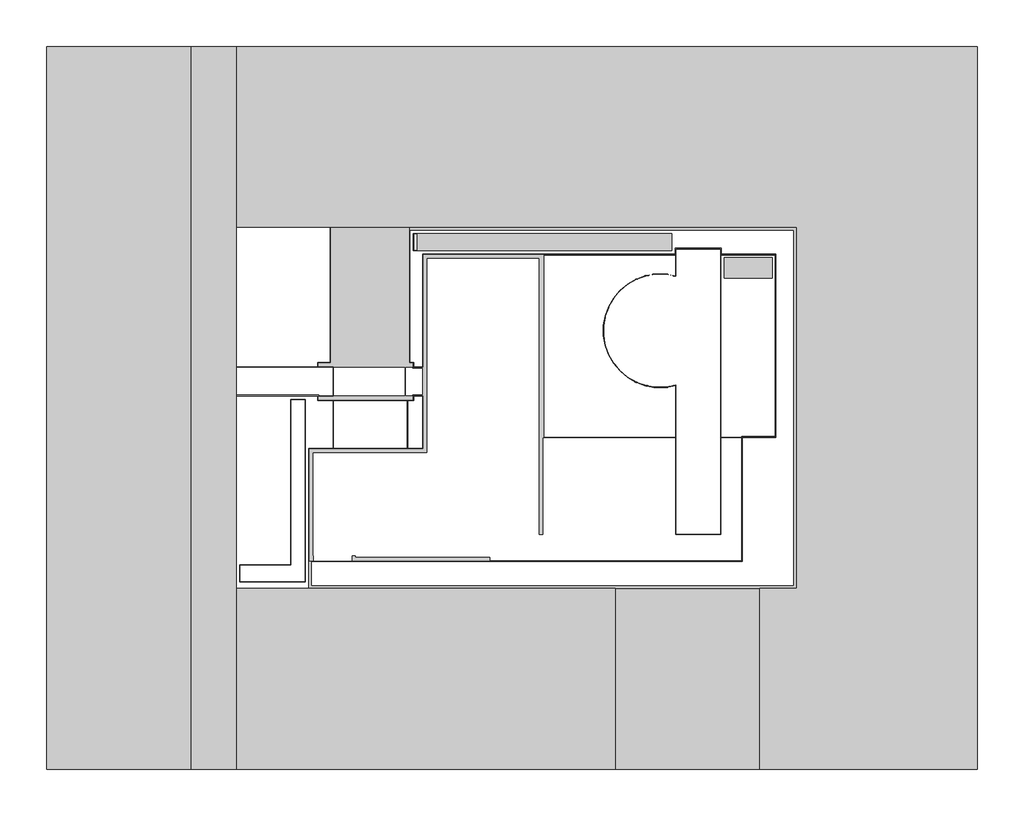
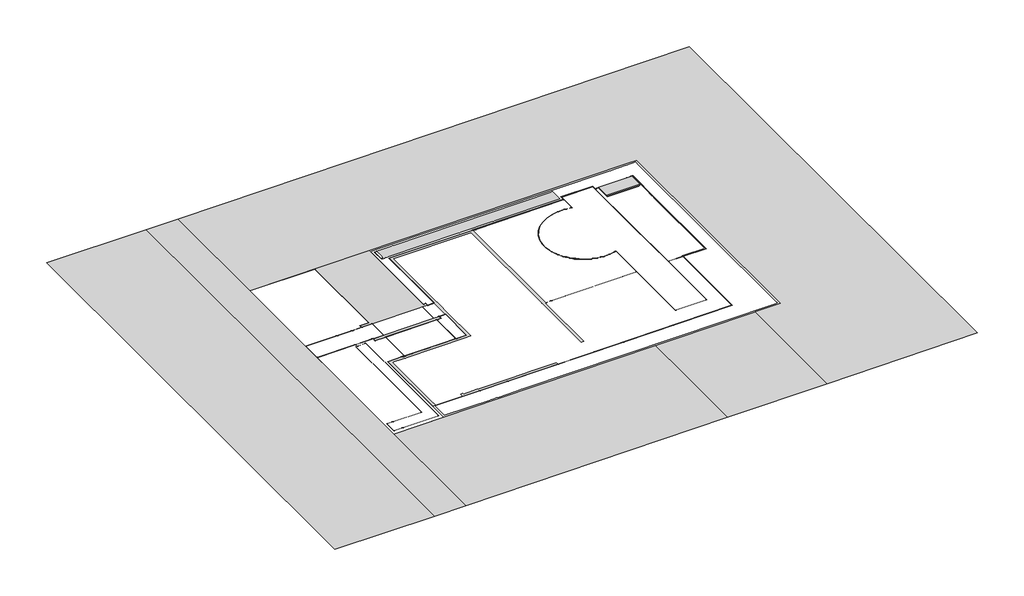
# One storey: 11 proxies.
"""IFC4 building model written with IfcOpenShell, lengths in millimetres."""

import ifcopenshell
import ifcopenshell.guid

model = None  # the IFC model being written
_history = None  # IfcOwnerHistory: only IFC2X3 demands one
_inside = {}  # id of a spatial element -> (the spatial element, [elements in it])
_under = {}  # id of a project, library or spatial element -> (it, [spatial elements below it])
_declared = {}  # id of a project -> (the project, [libraries it declares])
_typed = {}  # id of a type object -> (the type object, [elements of that type])
_made_of = {}  # id of a material, layer set ... -> (it, [elements and type objects made of it])


def new_model(schema):
    """Start an empty IFC model of exactly this schema.

    Asked for "IFC4X3", IfcOpenShell would pick the latest addendum, in which some entities
    have other attributes; the version numbers below select the first issue.
    IFC2X3 requires an IfcOwnerHistory on every rooted entity: one is made here for all.
    """
    global model, _history
    if schema == "IFC4X3":
        model = ifcopenshell.file(schema_version=(4, 3, 0, 0))
    else:
        model = ifcopenshell.file(schema=schema)
    _inside.clear()
    _under.clear()
    _declared.clear()
    _typed.clear()
    _made_of.clear()
    _history = None
    if model.schema == "IFC2X3":
        org = make("IfcOrganization", Name="unknown")
        user = make(
            "IfcPersonAndOrganization",
            ThePerson=make("IfcPerson", FamilyName="unknown"),
            TheOrganization=org,
        )
        app = make(
            "IfcApplication",
            ApplicationDeveloper=org,
            Version="unknown",
            ApplicationFullName="unknown",
            ApplicationIdentifier="unknown",
        )
        _history = make(
            "IfcOwnerHistory",
            OwningUser=user,
            OwningApplication=app,
            ChangeAction="ADDED",
            CreationDate=0,
        )
    return model


def make(cls, **values):
    """One entity of the class cls with the attributes given. An attribute that is None is left unset."""
    return model.create_entity(
        cls, **{name: value for name, value in values.items() if value is not None}
    )


def rooted(cls, **values):
    """An entity with a GlobalId (a new one), such as an element, a storey or a relation."""
    return make(cls, GlobalId=ifcopenshell.guid.new(), OwnerHistory=_history, **values)


def si_unit(unit_type, name, prefix=None):
    """IfcSIUnit, for example si_unit("LENGTHUNIT", "METRE", prefix="MILLI")."""
    return make("IfcSIUnit", UnitType=unit_type, Prefix=prefix, Name=name)


def assignment(units):
    """IfcUnitAssignment: the units of a project."""
    return None if units is None else make("IfcUnitAssignment", Units=units)


def point(xyz):
    """IfcCartesianPoint."""
    return None if xyz is None else make("IfcCartesianPoint", Coordinates=xyz)


def direction(xyz):
    """IfcDirection."""
    return None if xyz is None else make("IfcDirection", DirectionRatios=xyz)


def frame(location, z_axis=None, x_axis=None):
    """IfcAxis2Placement3D, a coordinate frame: its origin and axes. An axis left out is left unset."""
    return make(
        "IfcAxis2Placement3D",
        Location=point(location),
        Axis=direction(z_axis),
        RefDirection=direction(x_axis),
    )


def origin():
    """The frame at (0, 0, 0) with its axes left unset."""
    return frame((0.0, 0.0, 0.0))


def place(relative_to, where):
    """IfcLocalPlacement: puts the frame where relative to a parent placement (None: the world)."""
    return make(
        "IfcLocalPlacement", PlacementRelTo=relative_to, RelativePlacement=where
    )


def context(
    kind, dimensions, precision=None, world=None, true_north=None, identifier=None
):
    """IfcGeometricRepresentationContext, for example the 3D "Model" context."""
    return make(
        "IfcGeometricRepresentationContext",
        ContextIdentifier=identifier,
        ContextType=kind,
        CoordinateSpaceDimension=dimensions,
        Precision=precision,
        WorldCoordinateSystem=world,
        TrueNorth=true_north,
    )


def project(units=None, contexts=None):
    """IfcProject with its units and contexts."""
    return rooted(
        "IfcProject",
        Name="project",
        RepresentationContexts=contexts,
        UnitsInContext=assignment(units),
    )


def spatial(cls, under=None, at=None, **own):
    """A site, building, storey or space (cls), placed at a placement, below another one or the project."""
    s = rooted(cls, ObjectPlacement=at, **own)
    if under is not None:
        _under.setdefault(under.id(), (under, []))[1].append(s)
    return s


def polyline(points):
    """IfcPolyline through the points."""
    return make("IfcPolyline", Points=[point(p) for p in points])


def point_list(points):
    """IfcCartesianPointList2D or 3D."""
    cls = (
        "IfcCartesianPointList2D" if len(points[0]) == 2 else "IfcCartesianPointList3D"
    )
    return make(cls, CoordList=points)


def outline(outer, holes=None, kind="AREA"):
    """IfcArbitraryClosedProfileDef: a profile drawn as a closed curve; with holes, ...WithVoids."""
    if holes is None:
        return make("IfcArbitraryClosedProfileDef", ProfileType=kind, OuterCurve=outer)
    return make(
        "IfcArbitraryProfileDefWithVoids",
        ProfileType=kind,
        OuterCurve=outer,
        InnerCurves=holes,
    )


def extrude(swept, where, along, depth):
    """IfcExtrudedAreaSolid: the profile swept, set in the frame where, extruded along a direction by depth."""
    return make(
        "IfcExtrudedAreaSolid",
        SweptArea=swept,
        Position=where,
        ExtrudedDirection=direction(along),
        Depth=depth,
    )


def triangles(points, corners, closed=None, point_numbers=None):
    """IfcTriangulatedFaceSet: each triangle names its three corners, points numbered from 1."""
    return make(
        "IfcTriangulatedFaceSet",
        Coordinates=point_list(points),
        Closed=closed,
        CoordIndex=corners,
        PnIndex=point_numbers,
    )


def shape(context_of_items, identifier, shape_type, items):
    """IfcShapeRepresentation: the items that make up one representation, for example the "Body"."""
    return make(
        "IfcShapeRepresentation",
        ContextOfItems=context_of_items,
        RepresentationIdentifier=identifier,
        RepresentationType=shape_type,
        Items=items,
    )


def source(mapping_origin, context_of_items, identifier, shape_type, items):
    """IfcRepresentationMap: a shape defined once, which mapped items show again and again."""
    return make(
        "IfcRepresentationMap",
        MappingOrigin=mapping_origin,
        MappedRepresentation=shape(context_of_items, identifier, shape_type, items),
    )


def transform(
    local_origin,
    x_axis=None,
    y_axis=None,
    z_axis=None,
    scale=None,
    scale2=None,
    scale3=None,
    uniform=True,
):
    """IfcCartesianTransformationOperator3D, or its non-uniform kind. x_axis, y_axis, z_axis: its Axis1, 2, 3."""
    if uniform:
        return make(
            "IfcCartesianTransformationOperator3D",
            Axis1=direction(x_axis),
            Axis2=direction(y_axis),
            LocalOrigin=point(local_origin),
            Scale=scale,
            Axis3=direction(z_axis),
        )
    return make(
        "IfcCartesianTransformationOperator3DnonUniform",
        Axis1=direction(x_axis),
        Axis2=direction(y_axis),
        LocalOrigin=point(local_origin),
        Scale=scale,
        Axis3=direction(z_axis),
        Scale2=scale2,
        Scale3=scale3,
    )


def mapped(mapping_source, mapping_target):
    """IfcMappedItem: shows the shape of a source again, moved by a transform."""
    return make(
        "IfcMappedItem", MappingSource=mapping_source, MappingTarget=mapping_target
    )


def made_of(thing, what):
    """Note that an element or type object is made of a material, layer set ...; save() writes the relation."""
    if what is not None:
        _made_of.setdefault(what.id(), (what, []))[1].append(thing)
    return thing


def element(
    cls,
    number,
    at=None,
    inside=None,
    cuts=None,
    type_object=None,
    material=None,
    context=None,
    identifier="Body",
    shape_type=None,
    held_by="IfcProductDefinitionShape",
    body=None,
    shapes=None,
    **own,
):
    """One element of the class cls, such as IfcWall. Its Tag is "e" and its number.

    at: its placement. inside: the storey or other place that contains it. cuts: it is an
    opening in that element (IfcRelVoidsElement). A single representation is given by context,
    identifier, shape_type and body (its items); several are given by shapes. held_by: the class
    of the entity that holds the representations. save() writes the other relations.
    """
    e = rooted(cls, Tag="e%d" % number, ObjectPlacement=at, **own)
    if body is not None:
        shapes = [shape(context, identifier, shape_type, body)]
    if shapes is not None:
        e.Representation = make(held_by, Representations=shapes)
    if inside is not None:
        _inside.setdefault(inside.id(), (inside, []))[1].append(e)
    if cuts is not None:
        rooted(
            "IfcRelVoidsElement", RelatingBuildingElement=cuts, RelatedOpeningElement=e
        )
    if type_object is not None:
        _typed.setdefault(type_object.id(), (type_object, []))[1].append(e)
    return made_of(e, material)


def aggregate(whole, parts):
    """IfcRelAggregates: a whole, such as a stair, and the parts it consists of."""
    return rooted("IfcRelAggregates", RelatingObject=whole, RelatedObjects=parts)


def save(model, path):
    """Write the relations noted so far, then the file.

    IfcRelAggregates (storeys below a building ...), IfcRelContainedInSpatialStructure (elements
    in a storey), IfcRelDefinesByType, IfcRelAssociatesMaterial and IfcRelDeclares: one each for
    every whole, place, type object, material and project.
    """
    for whole, parts in _under.values():
        aggregate(whole, parts)
    for where, things in _inside.values():
        rooted(
            "IfcRelContainedInSpatialStructure",
            RelatedElements=things,
            RelatingStructure=where,
        )
    for kind, things in _typed.values():
        rooted("IfcRelDefinesByType", RelatedObjects=things, RelatingType=kind)
    for what, things in _made_of.values():
        rooted("IfcRelAssociatesMaterial", RelatedObjects=things, RelatingMaterial=what)
    for by, libraries in _declared.values():
        rooted("IfcRelDeclares", RelatingContext=by, RelatedDefinitions=libraries)
    model.write(path)


def specialty_equipment_67e2e29c(model_context):
    return source(origin(), model_context, "Body", "SweptSolid", [
        extrude(outline(polyline([(12687.718693, 5627.4300153), (12687.718693, 4481.4300153), (10041.718693, 4481.4300153), (10041.718693, 5627.4300153), (12687.718693, 5627.4300153)])), frame((0.0, 0.0, 280.0), z_axis=(0.0, 0.0, 1.0), x_axis=(1.0, 0.0, 0.0)), (0.0, 0.0, 1.0), 88.4706632),
        extrude(outline(polyline([(12614.718693, 5554.4300153), (12614.718693, 4554.4300153), (10114.718693, 4554.4300153), (10114.718693, 5554.4300153), (12614.718693, 5554.4300153)])), frame((0.0, 0.0, 200.0), z_axis=(0.0, 0.0, 1.0), x_axis=(1.0, 0.0, 0.0)), (0.0, 0.0, 1.0), 80.0),
    ])


model = new_model("IFC4")

# Units and contexts
model_context = context("Model", 3, world=origin())
ifc_project = project(units=[si_unit("LENGTHUNIT", "METRE", prefix="MILLI")], contexts=[model_context])

# Site, building, storey
site = spatial("IfcSite", under=ifc_project)
building = spatial("IfcBuilding", under=site)
storey = spatial("IfcBuildingStorey", under=building, Name="NÍVEL DA RUA", Elevation=0.0)

# Proxies
placement = place(None, origin())
element("IfcBuildingElementProxy", 1, Name="Building Element Proxy", at=placement, inside=storey, context=model_context, shape_type="Tessellation", body=[
    triangles([(-27460.2819946, 17304.4298035, 0.0), (-27460.2819946, -22695.5705017, 0.0), (-19460.2807709, -22695.5705017, 0.0), (-19460.2807709, -15076.5227692, 13.1362894), (-19460.2807709, 161.5728776, 13.1362894), (-19460.2807709, 9685.3826523, 13.1362894), (-19460.2807709, 17304.4298035, 0.0), (4007.9983795, -22695.5705017, 161.8502044), (4007.9983795, -16555.5790009, 161.8502044), (4007.9983795, -12695.5704254, 161.8502044), (-8585.2811966, -12695.5704254, 75.0000006), (-16960.2810425, -12695.5704254, 17.2413792), (-16960.2810425, -20396.7201233, 17.2413792), (-16960.2810425, -22695.5705017, 17.2413792), (-16960.2810425, 7304.4297272, 17.2413792), (13164.7185333, 7304.4297272, 225.0000017), (14039.7186127, 7304.4297272, 231.0344808), (14039.7186127, -12695.5704254, 231.0344808), (12007.9984406, -12695.5704254, 217.022618), (12007.9984406, -19007.6863037, 217.022618), (12007.9984406, -22695.5705017, 217.022618), (24039.718689, -22695.5705017, 300.0000023), (24039.718689, 17304.4298035, 300.0000023), (-16960.2810425, 17304.4298035, 17.2413792), (-16960.2810425, 16538.146344, 17.2413792)], [[2, 3, 4], [2, 4, 5], [13, 14, 11], [2, 5, 1], [1, 6, 7], [6, 1, 5], [16, 24, 25], [16, 25, 15], [8, 9, 11], [22, 18, 20], [18, 22, 17], [22, 20, 21], [19, 20, 18], [9, 10, 11], [12, 13, 11], [17, 23, 16], [22, 23, 17], [23, 24, 16], [11, 14, 8]], closed=False),
])
element("IfcBuildingElementProxy", 2, Name="Building Element Proxy", at=placement, inside=storey, context=model_context, shape_type="Tessellation", body=[
    triangles([(4007.9983795, -12695.5704254, 161.8502044), (4007.9983795, -16555.5790009, 161.8502044), (4007.9983795, -22695.5705017, 161.8502044), (12007.9984406, -22695.5705017, 217.022618), (12007.9984406, -19007.6863037, 217.022618), (12007.9984406, -12695.5704254, 217.022618)], [[2, 3, 5], [1, 2, 6], [4, 5, 3], [5, 6, 2]], closed=False),
])
element("IfcBuildingElementProxy", 3, Name="Building Element Proxy", at=placement, inside=storey, context=model_context, shape_type="Tessellation", body=[
    triangles([(-19460.2807709, -22695.5705017, 0.0), (-16960.2810425, -22695.5705017, 17.2413792), (-16960.2810425, -20396.7201233, 17.2413792), (-16960.2810425, -12695.5704254, 17.2413792), (-16960.2810425, 7304.4297272, 17.2413792), (-16960.2810425, 16538.146344, 17.2413792), (-16960.2810425, 17304.4298035, 17.2413792), (-19460.2807709, 17304.4298035, 0.0), (-19460.2807709, 9685.3826523, 13.1362894), (-19460.2807709, 161.5728776, 13.1362894), (-19460.2807709, -15076.5227692, 13.1362894)], [[10, 11, 4], [6, 8, 9], [5, 9, 10], [11, 1, 3], [11, 3, 4], [3, 1, 2], [6, 7, 8], [6, 9, 5], [4, 5, 10]], closed=False),
])
element("IfcBuildingElementProxy", 4, Name="Building Element Proxy", at=placement, inside=storey, context=model_context, shape_type="Tessellation", body=[
    triangles([(14039.7186127, 7304.4297272, 231.0344808), (13164.7185333, 7304.4297272, 225.0000017), (-7360.2815506, 7304.4297272, 83.4482767), (-7360.2815506, 7054.4298706, 83.4482767), (-7360.2815506, -195.5699849, 83.4482767), (-7160.2815491, -195.5699849, 84.8275893), (-7160.2815491, -445.5699686, 84.8275893), (-6660.2812546, -445.5699686, 88.2758617), (-6660.2812546, 5804.4300064, 88.2758617), (39.7186921, 5804.4300064, 134.4827615), (7339.7188522, 5804.4300064, 184.827581), (7339.7188522, 6104.4302994, 184.827581), (9839.719162, 6104.4302994, 202.0689704), (9839.719162, 5804.4300064, 202.0689704), (12414.7189636, 5804.4300064, 219.8275885), (12736.6074554, 5804.4300064, 222.0475111), (12889.7190399, 5804.4300064, 223.1034423), (12889.7190399, 5796.7827988, 223.1034423), (12889.7190399, 2838.5967934, 223.1034423), (12889.7190399, -4345.5699257, 223.1034423), (11039.7191711, -4345.5699257, 210.3448279), (11039.7191711, -11195.5701233, 210.3448279), (-6954.0313477, -11195.5701233, 86.2500043), (-9213.4062286, -11195.5701233, 70.668102), (-12960.281012, -11195.5701233, 44.8275872), (-12960.281012, -4945.5702209, 44.8275872), (-11830.5941528, -4945.5702209, 52.618536), (-11610.2808563, -4945.5702209, 54.1379291), (-11610.2808563, -4820.5615723, 54.1379291), (-11610.2808563, -2295.5700554, 54.1379291), (-12460.2812988, -2295.5700554, 48.2758642), (-12460.2812988, -2045.5700535, 48.2758642), (-13907.2197235, -2045.5700535, 38.296972), (-16960.2810425, -2045.5700535, 17.2413792), (-16960.2810425, -12695.5704254, 17.2413792), (-8585.2811966, -12695.5704254, 75.0000006), (14039.7186127, -12695.5704254, 231.0344808), (-12461.2812378, -2046.5183968, 48.2689651), (-12461.2812378, -2051.3699902, 48.2689651), (-12461.2812378, -2296.5699944, 48.2689651), (-12460.4696594, -2296.5699944, 48.2745606), (-11611.2807953, -2296.5699944, 54.1310346), (-11611.2807953, -4821.1289795, 54.1310346), (-11611.2807953, -4944.5697006, 54.1310346), (-11828.8314697, -4944.5697006, 52.6306901), (-11830.8313477, -4944.5697006, 52.6168964), (-12960.0926514, -4944.5697006, 44.8288862), (-12961.2809509, -4944.5697006, 44.8206881), (-12961.2809509, -4947.507312, 44.8206881), (-12961.2809509, -11195.944519, 44.8206881), (-12961.2809509, -12694.5704865, 44.8206881), (-16957.6149261, -12694.5704865, 17.2597704), (-16959.2811035, -12694.5704865, 17.2482761), (-16959.2811035, -12693.6321716, 17.2482761), (-16959.2811035, -2046.5183968, 17.2482761), (-13906.9104401, -2046.5183968, 38.2991112), (13889.7184662, 7154.430162, 230.0000054), (13889.7184662, 6721.9298172, 230.0000054), (13889.7184662, -12278.0703278, 230.0000054), (13889.7184662, -12545.5702789, 230.0000054), (13739.7183197, -12545.5702789, 228.9655118), (-6622.781218, -12545.5702789, 88.5344851), (-8422.1562698, -12545.5702789, 76.125), (-8648.0936417, -12545.5702789, 74.5668103), (-9022.7812363, -12545.5702789, 71.9827565), (-12809.2809265, -12545.5702789, 45.8689662), (-12809.2809265, -11247.3413818, 45.8689662), (-12809.2809265, -11196.5700623, 45.8689662), (-9212.9876495, -11196.5700623, 70.6709906), (-6955.119072, -11196.5700623, 86.2425011), (9.7186928, -11196.5700623, 134.275861), (2289.7186684, -11196.5700623, 150.0000011), (6259.7184952, -11196.5700623, 177.3793074), (11026.6350861, -11196.5700623, 210.25459), (11040.7191101, -11196.5700623, 210.3517316), (11040.7191101, -4348.353186, 210.3517316), (11040.7191101, -4346.5698647, 210.3517316), (12890.7189789, -4346.5698647, 223.110346), (12890.7189789, 2842.4799866, 223.110346), (12890.7189789, 5802.2650223, 223.110346), (12890.7189789, 5805.4299454, 223.110346), (12736.8923218, 5805.4299454, 222.0494732), (12415.2189331, 5805.4299454, 219.8310403), (9870.7184326, 5805.4299454, 202.2827655), (9870.7184326, 6135.4301514, 202.2827655), (7308.7184189, 6135.4301514, 184.6137859), (7308.7184189, 5805.4299454, 184.6137859), (48.468694, 5805.4299454, 134.5431049), (34.7853586, 5805.4299454, 134.4487338), (-6661.2811935, 5805.4299454, 88.2689672), (-6661.2811935, 5795.8584366, 88.2689672), (-6661.2811935, 5792.4301575, 88.2689672), (-6661.2811935, -444.5699933, 88.2689672), (-6662.2811325, -444.5699933, 88.2620726), (-7159.2810287, -444.5699933, 84.8344839), (-7159.2810287, -196.0699907, 84.8344839), (-7159.2810287, -194.5699914, 84.8344839), (-7160.1978333, -194.5699914, 84.8281616), (-7359.2810303, -194.5699914, 83.4551713), (-7359.2810303, -186.9985604, 83.4551713), (-7359.2810303, 7154.430162, 83.4551713), (-7290.2811722, 7154.430162, 83.9310325), (-6620.2813705, 7154.430162, 88.5517261), (11852.2184143, 7154.430162, 215.9482831), (13089.7184601, 7154.430162, 224.4827549), (13121.907193, 7154.430162, 224.7047436), (13137.3585754, 7154.430162, 224.8113141), (-12460.2812988, -445.5699686, 48.2758642), (-12460.2812988, -195.5699849, 48.2758642), (-11760.2810028, -195.5699849, 53.1034492), (-11760.2810028, 7054.4298706, 53.1034492), (-11760.2810028, 7304.4297272, 53.1034492), (-16960.2810425, 7304.4297272, 17.2413792), (-16960.2810425, -445.5699686, 17.2413792), (-14429.6692291, -445.5699686, 34.6938784), (-13230.3342957, -445.5699686, 42.9651464), (-11761.2809418, 7303.4297882, 53.0965501), (-11761.2809418, 7293.7158463, 53.0965501), (-11761.2809418, -194.5699914, 53.0965501), (-12460.1882813, -194.5699914, 48.2765046), (-12461.2812378, -194.5699914, 48.2689651), (-12461.2812378, -439.5699715, 48.2689651), (-12463.7648071, -439.5699715, 48.2518331), (-13233.2224915, -439.5699715, 42.9452348), (-14431.6284119, -439.5699715, 34.6803663), (-16959.2811035, -439.5699715, 17.2482761), (-16959.2811035, 7301.3677048, 17.2482761), (-16959.2811035, 7302.351947, 17.2482761), (-16959.2811035, 7303.4297882, 17.2482761), (-6660.2812546, -4945.5702209, 88.2758617), (-6660.2812546, -2045.5700535, 88.2758617), (-7160.2815491, -2045.5700535, 84.8275893), (-7160.2815491, -2295.5700554, 84.8275893), (-7510.2811157, -2295.5700554, 82.4137922), (-7510.2811157, -2494.1649101, 82.4137922), (-7510.2811157, -4945.5702209, 82.4137922), (-6661.2811935, -2046.5699924, 88.2689672), (-6661.2811935, -4940.2699631, 88.2689672), (-6661.2811935, -4944.5697006, 88.2689672), (-7484.2815399, -4944.5697006, 82.5931054), (-7484.2815399, -2479.4120316, 82.5931054), (-7484.2815399, -2296.5699944, 82.5931054), (-7162.0436508, -2296.5699944, 84.8154352), (-7160.0926071, -2296.5699944, 84.8288883), (-7159.2810287, -2296.5699944, 84.8344839), (-7159.2810287, -2295.0699406, 84.8344839), (-7159.2810287, -2046.5699924, 84.8344839), (-6662.2811325, -2046.5699924, 88.2620726), (-7159.2810287, 6005.4299469, 84.8344839), (-6960.2815475, 6005.4299469, 86.2068928), (-6960.2815475, 6447.2872787, 86.2068928), (-6960.2815475, 6953.4302216, 86.2068928), (-7159.2810287, 6953.4302216, 84.8344839), (-7159.2810287, 6873.7159012, 84.8344839), (7140.7187897, 6955.4300995, 183.455172), (-5638.5476898, 6955.4300995, 95.3222975), (-7161.281488, 6955.4300995, 84.8206856), (-7161.281488, 6878.0016861, 84.8206856), (-7161.281488, 6003.430069, 84.8206856), (-6753.1482605, 6003.430069, 87.635403), (-942.0146662, 6003.430069, 127.712181), (1780.9687626, 6003.430069, 146.4913763), (7140.7187897, 6003.430069, 183.455172), (7140.7187897, 6615.9729126, 183.455172), (-6960.2815475, 6954.4301605, 86.2068928), (-5633.6148514, 6954.4301605, 95.3563253), (7139.7188507, 6954.4301605, 183.4482684), (7139.7188507, 6615.8583847, 183.4482684), (7139.7188507, 6004.4300079, 183.4482684), (1789.7186646, 6004.4300079, 146.5517196), (-946.9479406, 6004.4300079, 127.6781623), (-6753.6145111, 6004.4300079, 87.6321874), (-6960.2815475, 6004.4300079, 86.2068928)], [[35, 53, 54], [53, 35, 52], [51, 52, 35], [35, 36, 51], [34, 35, 54], [66, 67, 50], [67, 25, 50], [25, 67, 68], [68, 24, 25], [66, 50, 51], [51, 65, 66], [49, 50, 25], [49, 26, 48], [49, 25, 26], [47, 48, 26], [26, 46, 47], [31, 41, 42], [39, 40, 31], [31, 40, 41], [30, 31, 42], [39, 32, 38], [46, 26, 27], [45, 46, 27], [68, 69, 24], [45, 28, 44], [45, 27, 28], [29, 44, 28], [65, 36, 64], [36, 65, 51], [64, 36, 63], [70, 24, 69], [36, 62, 63], [140, 135, 136], [43, 44, 29], [29, 30, 42], [31, 32, 39], [43, 29, 42], [140, 141, 135], [141, 142, 134], [142, 143, 133], [133, 143, 144], [142, 133, 134], [133, 147, 132], [141, 134, 135], [33, 55, 56], [55, 33, 34], [125, 114, 115], [55, 34, 54], [33, 38, 32], [123, 116, 108], [122, 108, 109], [115, 116, 124], [33, 56, 38], [108, 122, 123], [126, 127, 113], [113, 128, 129], [128, 113, 127], [113, 129, 112], [126, 113, 114], [115, 124, 125], [125, 126, 114], [123, 124, 116], [121, 109, 120], [121, 122, 109], [109, 119, 120], [5, 100, 4], [100, 5, 99], [99, 6, 98], [5, 6, 99], [119, 109, 110], [98, 6, 97], [154, 159, 149], [95, 6, 7], [118, 111, 112], [118, 112, 117], [117, 112, 129], [157, 158, 153], [154, 158, 159], [153, 158, 154], [157, 165, 156], [100, 101, 4], [101, 102, 3], [101, 3, 4], [102, 103, 3], [119, 110, 111], [153, 165, 157], [119, 111, 118], [133, 144, 145], [146, 147, 133], [130, 140, 136], [24, 70, 23], [139, 140, 130], [138, 139, 130], [131, 137, 138], [23, 71, 72], [148, 137, 131], [7, 94, 95], [7, 8, 94], [97, 6, 96], [95, 96, 6], [147, 148, 132], [94, 8, 93], [93, 8, 92], [91, 92, 9], [8, 9, 92], [91, 9, 90], [148, 131, 132], [70, 71, 23], [73, 22, 72], [22, 76, 21], [74, 75, 22], [61, 37, 60], [60, 37, 59], [22, 75, 76], [58, 59, 37], [37, 61, 62], [73, 74, 22], [131, 138, 130], [87, 10, 11], [89, 9, 10], [21, 77, 20], [21, 76, 77], [20, 78, 19], [19, 78, 79], [18, 79, 80], [18, 19, 79], [78, 20, 77], [17, 18, 80], [58, 37, 1], [23, 72, 22], [62, 36, 37], [90, 9, 89], [160, 173, 159], [172, 150, 173], [172, 173, 160], [152, 166, 165], [161, 171, 160], [149, 159, 173], [156, 165, 166], [89, 10, 88], [162, 163, 170], [163, 169, 170], [170, 171, 162], [87, 88, 10], [162, 171, 161], [172, 171, 166], [170, 166, 171], [149, 173, 150], [160, 171, 172], [165, 153, 152], [166, 151, 172], [151, 150, 172], [168, 167, 170], [169, 163, 164], [170, 167, 166], [166, 155, 156], [167, 155, 166], [167, 168, 164], [152, 151, 166], [168, 170, 169], [11, 12, 87], [84, 13, 14], [12, 13, 86], [13, 85, 86], [13, 84, 85], [168, 169, 164], [17, 82, 16], [15, 16, 83], [16, 82, 83], [82, 17, 81], [80, 81, 17], [84, 15, 83], [104, 105, 2], [2, 3, 104], [164, 155, 167], [106, 107, 2], [2, 57, 1], [57, 2, 107], [1, 57, 58], [106, 2, 105], [103, 104, 3], [87, 12, 86], [15, 84, 14], [133, 145, 146]], closed=False),
])
element("IfcBuildingElementProxy", 5, Name="Building Element Proxy", at=placement, inside=storey, context=model_context, shape_type="Tessellation", body=[
    triangles([(-7510.2811157, -2295.5700554, 82.4137922), (-11610.2808563, -2295.5700554, 54.1379291), (-11610.2808563, -4820.5615723, 54.1379291), (-11610.2808563, -4945.5702209, 54.1379291), (-7510.2811157, -4945.5702209, 82.4137922), (-7510.2811157, -2494.1649101, 82.4137922), (-7511.2810547, -2296.5699944, 82.4068977), (-7511.2810547, -2494.1163666, 82.4068977), (-7511.2810547, -4944.5697006, 82.4068977), (-7543.0791138, -4944.5697006, 82.1875978), (-11609.2809174, -4944.5697006, 54.1448282), (-11609.2809174, -4820.5920937, 54.1448282), (-11609.2809174, -2296.5699944, 54.1448282), (-11589.6367676, -2296.5699944, 54.2803123)], [[3, 4, 11], [11, 4, 10], [3, 11, 12], [2, 3, 13], [13, 14, 2], [13, 3, 12], [2, 14, 1], [10, 5, 9], [5, 10, 4], [9, 5, 6], [9, 6, 8], [7, 8, 6], [6, 1, 7], [7, 1, 14]], closed=False),
])
element("IfcBuildingElementProxy", 6, Name="Building Element Proxy", at=placement, inside=storey, context=model_context, shape_type="Tessellation", body=[
    triangles([(7339.7188522, -4345.5699257, 184.827581), (7339.7188522, -9695.5698212, 184.827581), (9839.719162, -9695.5698212, 202.0689704), (9839.719162, -4345.5699257, 202.0689704), (9839.719162, 654.4300398, 202.0689704), (9839.719162, 6104.4302994, 202.0689704), (7339.7188522, 6104.4302994, 184.827581), (7339.7188522, 4607.5800957, 184.827581), (6796.6921143, 4709.4366692, 181.0825697), (6244.2217667, 4714.8491295, 177.272428), (5699.3044464, 4623.6503357, 173.5143907), (5178.7025024, 4438.6465118, 169.9240212), (4698.432399, 4165.5288803, 166.6118142), (4273.2688156, 3812.6995445, 163.6796531), (3916.2914772, 3391.0127838, 161.2177394), (3638.4822716, 2913.4410622, 159.3018135), (3448.3874794, 2394.6766514, 157.9908106), (3351.8552902, 1850.6783157, 157.3250809), (3351.8552902, 1298.1816616, 157.3250809), (3375.1727623, 1166.7781271, 157.4858814), (3448.3874794, 754.1833986, 157.9908106), (3638.4822716, 235.4189333, 159.3018135), (3916.2914772, -242.152643, 161.2177394), (4273.2688156, -663.8394218, 163.6796531), (4698.432399, -1016.6688303, 166.6118142), (5116.5376923, -1254.4350586, 169.4953046), (5178.7025024, -1289.7865345, 169.9240212), (5699.3044464, -1474.7903584, 173.5143907), (6244.2217667, -1565.9890068, 177.272428), (6796.6921143, -1560.5766918, 181.0825697), (7339.7188522, -1458.7201183, 184.827581), (9838.719223, 6103.4297791, 202.0620668), (9838.719223, 656.0112659, 202.0620668), (9838.719223, 653.5847425, 202.0620668), (9838.719223, -4344.415345, 202.0620668), (9838.719223, -4345.5699257, 202.0620668), (9838.719223, -4347.7099113, 202.0620668), (9838.719223, -9694.5698822, 202.0620668), (7340.7187912, -9694.5698822, 184.8344846), (7340.7187912, -9693.4298355, 184.8344846), (7340.7187912, -4345.5699257, 184.8344846), (7340.7187912, -1459.8748444, 184.8344846), (7340.7187912, -1457.8749664, 184.8344846), (7340.7187912, -1447.0134201, 184.8344846), (7339.7188522, -1447.2022167, 184.827581), (7298.6940308, -1454.9504356, 184.5446586), (6799.331488, -1549.2634289, 181.1007736), (6738.2637039, -1549.930394, 180.6796147), (6248.4058136, -1555.2806488, 177.3012962), (6140.4943771, -1537.3313084, 176.5570647), (5704.9145691, -1464.8797714, 173.5530693), (5198.0809708, -1285.2682056, 170.0576795), (5185.6009186, -1280.8455105, 169.9716019), (5184.0382233, -1279.9583553, 169.9608285), (5160.4478027, -1266.5664402, 169.7981386), (5149.7327591, -1260.4835266, 169.7242332), (5143.4308182, -1256.906274, 169.6807766), (5120.5310532, -1243.9063408, 169.5228466), (5100.9851532, -1232.8106518, 169.3880437), (5070.1288971, -1215.2939157, 169.1752479), (5020.0999741, -1186.8933964, 168.8302108), (4706.4641762, -1008.8477234, 166.6672069), (4382.4897652, -740.3338079, 164.4328956), (4282.2644875, -657.2659132, 163.7416951), (3966.0765198, -284.1410139, 161.5610869), (3926.0708221, -236.9313229, 161.2851771), (3891.4450287, -177.4590991, 161.0463836), (3648.8563477, 239.2065837, 159.3733571), (3598.8945717, 375.4450702, 159.0287923), (3459.1615311, 756.4792614, 158.0651157), (3405.0970985, 1060.9314629, 157.6922642), (3395.8714989, 1112.8837423, 157.6286416), (3389.9497673, 1146.2321428, 157.5878011), (3384.815197, 1175.1465843, 157.5523926), (3384.5727699, 1176.5109632, 157.5507212), (3384.2972054, 1178.0621767, 157.5488136), (3383.976004, 1179.8718773, 157.5465972), (3383.5896904, 1182.0475439, 157.5439447), (3383.1077431, 1184.7605324, 157.5406201), (3382.4787117, 1188.3028307, 157.5362781), (3381.6055092, 1193.2199724, 157.5302464), (3380.2823341, 1200.6721338, 157.5211264), (3377.9699753, 1213.692778, 157.5051753), (3372.528447, 1244.3365471, 157.4676594), (3362.8302017, 1298.9508007, 157.4007667), (3362.8302017, 1528.7872078, 157.4007667), (3362.8302017, 1849.9091766, 157.4007667), (3442.7352081, 2299.8790947, 157.9518414), (3459.1615311, 2392.3808613, 158.0651157), (3630.2714355, 2858.9754913, 159.2451854), (3648.8563477, 2909.6535027, 159.3733571), (3907.090004, 3353.1906738, 161.1542803), (3926.0708221, 3385.7913002, 161.2851771), (4263.5359795, 3784.025132, 163.6125242), (4282.2644875, 3806.1258179, 163.7416951), (4688.3600487, 4142.702948, 166.5423599), (4706.4641762, 4157.7078461, 166.6672069), (5168.3874344, 4419.9337006, 169.8528955), (5185.6009186, 4429.7054878, 169.9716019), (5688.8021805, 4608.0297775, 173.4419569), (5704.9145691, 4613.7398941, 173.5530693), (6233.5671844, 4701.6726082, 177.1989587), (6248.4058136, 4704.1407715, 177.3012962), (6785.9073074, 4698.2701996, 181.008192), (6799.331488, 4698.1234062, 181.1007736), (7328.8195175, 4598.1207893, 184.752422), (7335.6423569, 4596.8322052, 184.7994759), (7339.7188522, 4596.0621941, 184.827581), (7340.7187912, 4595.8732521, 184.8344846), (7340.7187912, 4605.9987968, 184.8344846), (7340.7187912, 4608.1788963, 184.8344846), (7340.7187912, 6103.4297791, 184.8344846)], [[21, 69, 70], [69, 21, 22], [21, 70, 71], [23, 67, 22], [22, 68, 69], [68, 22, 67], [20, 75, 76], [75, 20, 74], [20, 76, 77], [71, 72, 20], [73, 74, 20], [72, 73, 20], [20, 21, 71], [67, 23, 66], [60, 61, 26], [59, 60, 26], [56, 57, 26], [26, 58, 59], [58, 26, 57], [56, 26, 27], [61, 25, 26], [23, 65, 66], [65, 23, 24], [65, 24, 64], [25, 62, 63], [62, 25, 61], [64, 24, 63], [63, 24, 25], [84, 20, 83], [83, 20, 82], [79, 20, 78], [81, 20, 80], [80, 20, 79], [20, 81, 82], [87, 18, 86], [86, 18, 19], [18, 87, 88], [84, 85, 19], [85, 86, 19], [20, 84, 19], [18, 88, 17], [78, 20, 77], [17, 89, 90], [89, 17, 88], [17, 90, 16], [16, 91, 92], [91, 16, 90], [16, 92, 15], [15, 92, 93], [15, 94, 14], [15, 93, 94], [14, 94, 95], [96, 13, 14], [13, 97, 98], [97, 13, 96], [96, 14, 95], [28, 29, 50], [50, 29, 49], [51, 28, 50], [29, 48, 49], [48, 29, 30], [47, 48, 30], [30, 46, 47], [27, 52, 53], [27, 28, 52], [27, 53, 54], [46, 30, 31], [45, 46, 31], [31, 43, 45], [28, 51, 52], [2, 39, 40], [39, 2, 38], [1, 2, 40], [38, 3, 37], [3, 38, 2], [37, 4, 36], [4, 37, 3], [42, 43, 31], [42, 1, 41], [43, 44, 45], [41, 1, 40], [36, 4, 35], [1, 42, 31], [35, 4, 5], [55, 56, 27], [98, 99, 12], [98, 12, 13], [100, 11, 12], [100, 12, 99], [55, 27, 54], [11, 100, 101], [11, 102, 10], [11, 101, 102], [10, 102, 103], [104, 105, 9], [104, 10, 103], [10, 104, 9], [105, 106, 9], [8, 106, 107], [108, 110, 107], [34, 5, 33], [5, 34, 35], [5, 6, 33], [110, 108, 109], [110, 8, 107], [111, 8, 110], [112, 8, 111], [8, 112, 7], [6, 7, 32], [6, 32, 33], [32, 7, 112], [9, 106, 8]], closed=False),
])
element("IfcBuildingElementProxy", 7, Name="Building Element Proxy", at=placement, inside=storey, context=model_context, shape_type="Tessellation", body=[
    triangles([(39.7186921, 5804.4300064, 134.4827615), (39.7186921, -4345.5699257, 134.4827615), (495.343711, -4345.5699257, 137.6250025), (7339.7188522, -4345.5699257, 184.827581), (7339.7188522, -1458.7201183, 184.827581), (6796.6921143, -1560.5766918, 181.0825697), (6244.2217667, -1565.9890068, 177.272428), (5699.3044464, -1474.7903584, 173.5143907), (5178.7025024, -1289.7865345, 169.9240212), (5116.5376923, -1254.4350586, 169.4953046), (4698.432399, -1016.6688303, 166.6118142), (4273.2688156, -663.8394218, 163.6796531), (3916.2914772, -242.152643, 161.2177394), (3638.4822716, 235.4189333, 159.3018135), (3448.3874794, 754.1833986, 157.9908106), (3375.1727623, 1166.7781271, 157.4858814), (3351.8552902, 1298.1816616, 157.3250809), (3351.8552902, 1850.6783157, 157.3250809), (3448.3874794, 2394.6766514, 157.9908106), (3638.4822716, 2913.4410622, 159.3018135), (3916.2914772, 3391.0127838, 161.2177394), (4273.2688156, 3812.6995445, 163.6796531), (4698.432399, 4165.5288803, 166.6118142), (5178.7025024, 4438.6465118, 169.9240212), (5699.3044464, 4623.6503357, 173.5143907), (6244.2217667, 4714.8491295, 177.272428), (6796.6921143, 4709.4366692, 181.0825697), (7339.7188522, 4607.5800957, 184.827581), (7339.7188522, 5804.4300064, 184.827581), (7338.7189133, -1460.0386425, 184.8206955), (7338.7189133, -4340.4414597, 184.8206955), (7338.7189133, -4343.0325806, 184.8206955), (7338.7189133, -4344.5699867, 184.8206955), (496.8763209, -4344.5699867, 137.6355669), (496.0298246, -4344.5699867, 137.6297351), (40.7045512, -4344.5699867, 134.4895562), (40.7045512, 5754.4301514, 134.4895562), (76.4691787, 5754.4301514, 134.7362072), (81.6046937, 5754.4301514, 134.7716247), (89.7027914, 5754.4301514, 134.8274807), (101.9597376, 5754.4301514, 134.9120049), (120.031636, 5754.4301514, 135.0366431), (145.9968752, 5754.4301514, 135.215711), (181.8478755, 5754.4301514, 135.4629615), (227.8518807, 5754.4301514, 135.7802296), (7260.6062393, 5754.4301514, 184.2819747), (7270.2556503, 5754.4301514, 184.3485223), (7289.4475021, 5754.4301514, 184.4808907), (7314.9226913, 5754.4301514, 184.6565885), (7338.7189133, 5754.4301514, 184.8206955), (7338.7189133, 4608.8986198, 184.8206955), (6797.103717, 4710.266851, 181.085422), (6795.6020645, 4710.5479385, 181.0750666), (6245.1211304, 4715.743261, 177.2786413), (6243.0799759, 4715.7624458, 177.2645615), (5700.982251, 4624.8584015, 173.5259634), (5698.1417267, 4624.3819771, 173.5063607), (5182.2540298, 4440.8911423, 169.9485291), (5177.5438522, 4439.2159538, 169.9160457), (4697.2955498, 4165.9585052, 166.603984), (4272.1636505, 3813.0123161, 163.6720409), (3915.2211937, 3391.2302124, 161.2103634), (3637.4436722, 2913.5820419, 159.2946555), (3447.3730064, 2394.755135, 157.9838161), (3351.0251083, 1851.6695343, 157.3193582), (3350.8536072, 1850.7034595, 157.3181773), (3350.8536072, 1299.5445145, 157.3181773), (3350.8536072, 1298.1565178, 157.3181773), (3351.082663, 1296.8651722, 157.3197578), (3374.3905426, 1165.4854734, 157.4805038), (3447.3730064, 754.104915, 157.9838161), (3447.7136833, 753.1751026, 157.9861779), (3637.4436722, 235.2780444, 159.2946555), (3637.8384155, 234.5993068, 159.2973806), (3915.2211937, -242.3702169, 161.2103634), (4272.1636505, -664.1523388, 163.6720409), (4697.2955498, -1017.0985279, 166.603984), (5115.5615891, -1255.0883617, 169.4885645), (5177.5438522, -1290.3559765, 169.9160457), (5179.6297714, -1291.0977917, 169.9304162), (5698.1417267, -1475.5218544, 173.5063607), (5699.8898758, -1475.8150051, 173.5184239), (6243.0799759, -1566.9026138, 177.2645615), (6244.5763962, -1566.8883705, 177.2748806), (6795.6020645, -1561.6879612, 181.0750666), (6796.8630341, -1561.4520744, 181.0837506), (9839.719162, -4345.5699257, 202.0689704), (11039.7191711, -4345.5699257, 210.3448279), (12889.7190399, -4345.5699257, 223.1034423), (12889.7190399, 2838.5967934, 223.1034423), (12889.7190399, 5796.7827988, 223.1034423), (12889.7190399, 5804.4300064, 223.1034423), (12736.6074554, 5804.4300064, 222.0475111), (12414.7189636, 5804.4300064, 219.8275885), (9839.719162, 5804.4300064, 202.0689704), (9839.719162, 654.4300398, 202.0689704), (12839.7186035, 5754.4301514, 222.7586233), (12839.7186035, 3807.1167458, 222.7586233), (12839.7186035, 3150.7896561, 222.7586233), (12839.7186035, 2887.2167908, 222.7586233), (12839.7186035, 2802.7905487, 222.7586233), (12839.7186035, -4263.6028358, 222.7586233), (12839.7186035, -4295.5700706, 222.7586233), (11027.7187408, -4295.5700706, 210.262075), (10989.7187347, -4295.5700706, 210.0000089), (10989.7187347, -4344.5699867, 210.0000089), (9840.719101, -4344.5699867, 202.0758559), (9840.719101, 650.263361, 202.0758559), (9840.719101, 652.7906776, 202.0758559), (9840.719101, 655.1461298, 202.0758559), (9840.719101, 5754.4301514, 202.0758559), (9891.1381165, 5754.4301514, 202.4235818), (12422.7266144, 5754.4301514, 219.8828177), (12739.1886932, 5754.4301514, 222.0653153)], [[2, 3, 36], [36, 3, 35], [36, 37, 2], [34, 35, 3], [15, 72, 14], [68, 69, 17], [17, 69, 16], [68, 17, 67], [71, 15, 70], [15, 71, 72], [70, 16, 69], [16, 70, 15], [73, 14, 72], [11, 77, 78], [10, 78, 79], [10, 11, 78], [9, 80, 8], [79, 9, 10], [9, 79, 80], [14, 74, 13], [13, 74, 75], [74, 14, 73], [77, 12, 76], [12, 77, 11], [12, 13, 76], [76, 13, 75], [34, 3, 4], [44, 45, 1], [43, 44, 1], [67, 18, 66], [67, 17, 18], [65, 66, 18], [19, 65, 18], [1, 37, 38], [37, 1, 2], [1, 38, 39], [41, 42, 1], [39, 40, 1], [41, 1, 40], [1, 42, 43], [1, 45, 29], [64, 19, 63], [19, 64, 65], [63, 19, 20], [20, 21, 62], [61, 21, 22], [21, 61, 62], [20, 62, 63], [22, 60, 61], [59, 23, 24], [59, 60, 23], [22, 23, 60], [24, 58, 59], [58, 24, 25], [57, 25, 56], [25, 57, 58], [81, 8, 80], [83, 84, 7], [85, 7, 84], [83, 7, 8], [33, 4, 32], [4, 33, 34], [31, 32, 4], [4, 5, 31], [82, 83, 8], [8, 81, 82], [7, 85, 6], [6, 86, 30], [86, 6, 85], [30, 5, 6], [30, 31, 5], [107, 108, 87], [87, 106, 107], [106, 87, 88], [96, 87, 108], [88, 89, 103], [103, 104, 88], [89, 102, 103], [88, 104, 106], [105, 106, 104], [96, 109, 110], [109, 96, 108], [110, 111, 96], [101, 102, 90], [102, 89, 90], [26, 27, 53], [56, 25, 26], [26, 53, 54], [56, 26, 55], [51, 28, 50], [28, 51, 27], [27, 52, 53], [52, 27, 51], [54, 55, 26], [29, 47, 48], [48, 49, 29], [29, 46, 47], [29, 49, 50], [112, 113, 94], [111, 112, 95], [100, 90, 99], [96, 111, 95], [98, 99, 90], [90, 91, 98], [29, 50, 28], [93, 94, 113], [95, 112, 94], [97, 92, 93], [91, 92, 97], [97, 98, 91], [97, 93, 114], [93, 113, 114], [90, 100, 101], [46, 29, 45]], closed=False),
])
element("IfcBuildingElementProxy", 8, Name="Building Element Proxy", at=placement, inside=storey, context=model_context, shape_type="Tessellation", body=[
    triangles([(-12460.2812988, -2045.5700535, 48.2758642), (-11610.2808563, -2045.5700535, 54.1379291), (-11610.2808563, -445.5699686, 54.1379291), (-12460.2812988, -445.5699686, 48.2758642), (-13230.3342957, -445.5699686, 42.9651464), (-14429.6692291, -445.5699686, 34.6938784), (-16960.2810425, -445.5699686, 17.2413792), (-16960.2810425, -2045.5700535, 17.2413792), (-13907.2197235, -2045.5700535, 38.296972), (-11611.2807953, -446.5699802, 54.1310346), (-11611.2807953, -2043.6876102, 54.1310346), (-11611.2807953, -2044.5699692, 54.1310346), (-12410.2808624, -2044.5699692, 48.6206878), (-12410.2808624, -1994.5699688, 48.6206878), (-12460.2812988, -1994.5699688, 48.2758642), (-12484.8263123, -1994.5699688, 48.106584), (-13885.6442963, -1994.5699688, 38.4457729), (-13923.8733582, -1994.5699688, 38.1821262), (-16879.6185242, -1994.5699688, 17.7976782), (-16958.2811646, -1994.5699688, 17.2551729), (-16958.2811646, -446.5699802, 17.2551729), (-14431.250528, -446.5699802, 34.6829688), (-14429.3425049, -446.5699802, 34.6961289), (-13230.7575256, -446.5699802, 42.9622305), (-13229.8529297, -446.5699802, 42.9684665), (-12460.2812988, -446.5699802, 48.2758642)], [[8, 19, 20], [19, 8, 9], [8, 20, 7], [18, 9, 17], [9, 18, 19], [6, 7, 21], [21, 7, 20], [6, 21, 22], [23, 24, 6], [5, 6, 24], [5, 24, 25], [23, 6, 22], [16, 17, 9], [15, 1, 13], [13, 1, 2], [15, 13, 14], [11, 12, 2], [2, 12, 13], [11, 2, 3], [15, 16, 1], [26, 10, 4], [3, 4, 10], [26, 4, 25], [11, 3, 10], [25, 4, 5], [1, 16, 9]], closed=False),
])
element("IfcBuildingElementProxy", 9, Name="Building Element Proxy", at=placement, inside=storey, context=model_context, shape_type="Tessellation", body=[
    triangles([(-13160.2815948, -12345.569696, 43.4482746), (-13160.2815948, -11270.5701965, 43.4482746), (-13160.2815948, -5333.0698242, 43.4482746), (-13160.2815948, -4333.0701073, 43.4482746), (-13160.2815948, -2245.570055, 43.4482746), (-13841.9144073, -2245.570055, 38.7473624), (-13960.281601, -2245.570055, 37.9310355), (-13960.281601, -6883.0699814, 37.9310355), (-13960.281601, -11395.5695435, 37.9310355), (-13961.1536407, -11395.5695435, 37.9250152), (-16289.313858, -11395.5695435, 21.8687437), (-16760.2816223, -11395.5695435, 18.6206896), (-16760.2816223, -12308.0696594, 18.6206896), (-16760.2816223, -12345.569696, 18.6206896), (-16026.9484772, -12345.569696, 23.6781605), (-13958.7863434, -11396.5694824, 37.9413433), (-13958.7863434, -11395.3369995, 37.9413433), (-13958.7863434, -6891.2677368, 37.9413433), (-13958.7863434, -6880.1742279, 37.9413433), (-13958.7863434, -6878.3057373, 37.9413433), (-13958.7863434, -2249.470253, 37.9413433), (-13958.7863434, -2246.569994, 37.9413433), (-13841.5876831, -2246.569994, 38.7496151), (-13161.2815338, -2246.569994, 43.44138), (-13161.2815338, -4330.0075035, 43.44138), (-13161.2815338, -4336.2574127, 43.44138), (-13161.2815338, -5335.0074966, 43.44138), (-13161.2815338, -11265.0856476, 43.44138), (-13161.2815338, -11270.726001, 43.44138), (-13161.2815338, -11564.8638611, 43.44138), (-13161.2815338, -12344.5697571, 43.44138), (-16024.7730286, -12344.5697571, 23.6931645), (-16027.2240417, -12344.5697571, 23.6762551), (-16046.5030975, -12344.5697571, 23.543294), (-16759.2816833, -12344.5697571, 18.6275864), (-16759.2816833, -12308.1208191, 18.6275864), (-16759.2816833, -12306.1325684, 18.6275864), (-16759.2816833, -11396.5694824, 18.6275864), (-16289.8301056, -11396.5694824, 21.8651829), (-16289.0371307, -11396.5694824, 21.8706468), (-13962.4570496, -11396.5694824, 37.9160314)], [[14, 35, 13], [35, 14, 34], [13, 36, 37], [36, 13, 35], [12, 13, 37], [34, 15, 33], [15, 34, 14], [32, 33, 15], [12, 37, 38], [39, 40, 11], [11, 12, 38], [11, 40, 41], [11, 41, 10], [11, 38, 39], [9, 18, 8], [9, 10, 41], [7, 8, 20], [19, 8, 18], [17, 18, 9], [9, 41, 16], [32, 15, 1], [20, 21, 7], [17, 9, 16], [31, 1, 30], [1, 31, 32], [29, 30, 2], [2, 30, 1], [29, 2, 28], [3, 28, 2], [22, 23, 6], [6, 23, 24], [22, 6, 7], [22, 7, 21], [26, 3, 4], [3, 26, 27], [26, 4, 25], [25, 5, 24], [5, 25, 4], [24, 5, 6], [27, 28, 3], [8, 19, 20]], closed=False),
])
element("IfcBuildingElementProxy", 10, Name="Building Element Proxy", at=placement, inside=storey, context=model_context, shape_type="Tessellation", body=[
    triangles([(-7360.2815506, 7304.4297272, 83.4482767), (-11760.2810028, 7304.4297272, 53.1034492), (-11760.2810028, -195.5699849, 53.1034492), (-12460.2812988, -195.5699849, 48.2758642), (-12460.2812988, -445.5699686, 48.2758642), (-11610.2808563, -445.5699686, 54.1379291), (-11610.2808563, -2045.5700535, 54.1379291), (-12460.2812988, -2045.5700535, 48.2758642), (-12460.2812988, -2295.5700554, 48.2758642), (-7160.2815491, -2295.5700554, 84.8275893), (-7160.2815491, -2045.5700535, 84.8275893), (-6660.2812546, -2045.5700535, 88.2758617), (-6660.2812546, -4945.5702209, 88.2758617), (-11830.5941528, -4945.5702209, 52.618536), (-12960.281012, -4945.5702209, 44.8275872), (-12960.281012, -11195.5701233, 44.8275872), (-9213.4062286, -11195.5701233, 70.668102), (-6954.0313477, -11195.5701233, 86.2500043), (11039.7191711, -11195.5701233, 210.3448279), (11039.7191711, -4345.5699257, 210.3448279), (9839.719162, -4345.5699257, 202.0689704), (9839.719162, -9695.5698212, 202.0689704), (7339.7188522, -9695.5698212, 184.827581), (7339.7188522, -4345.5699257, 184.827581), (495.343711, -4345.5699257, 137.6250025), (39.7186921, -4345.5699257, 134.4827615), (39.7186921, 5804.4300064, 134.4827615), (-6660.2812546, 5804.4300064, 88.2758617), (-6660.2812546, -445.5699686, 88.2758617), (-7160.2815491, -445.5699686, 84.8275893), (-7160.2815491, -195.5699849, 84.8275893), (-7360.2815506, -195.5699849, 83.4482767), (-7610.2814072, -446.5699802, 81.7241359), (-7610.2814072, -2044.5699692, 81.7241359), (-11607.9844849, -2044.5699692, 54.1537757), (-11609.2809174, -2044.5699692, 54.1448282), (-11609.2809174, -446.5699802, 54.1448282), (-7936.9027496, -446.5699802, 79.4715754), (-7209.2814651, -446.5699802, 84.4896557), (-7209.2814651, -495.569969, 84.4896557), (-7160.2815491, -495.569969, 84.8275893), (-6675.9064636, -495.569969, 88.1681012), (-6661.2811935, -495.569969, 88.2689672), (-6661.2811935, -1995.5700531, 88.2689672), (-7144.65634, -1995.5700531, 84.9353407), (-7160.2815491, -1995.5700531, 84.8275893), (-7165.6864517, -1995.5700531, 84.7903096), (-7209.2814651, -1995.5700531, 84.4896557), (-7209.2814651, -2044.5699692, 84.4896557), (-7609.2814682, -2044.5699692, 81.7310305), (-7609.2814682, -446.5699802, 81.7310305), (-7333.1459976, -446.5699802, 83.635411), (-6440.281311, -5165.5701645, 89.793102), (-6440.281311, -4925.8685165, 89.793102), (-6440.281311, -2121.0923332, 89.793102), (-6440.281311, -573.6297029, 89.793102), (-6440.281311, -240.3461035, 89.793102), (-6440.281311, 5584.4300629, 89.793102), (-241.2813117, 5584.4300629, 132.5448257), (-210.2813144, 5584.4300629, 132.7586208), (-210.2813144, 5571.2209854, 132.7586208), (-210.2813144, -4200.0477036, 132.7586208), (-210.2813144, -4259.7490013, 132.7586208), (-210.2813144, -4367.958094, 132.7586208), (-210.2813144, -4590.4314331, 132.7586208), (-210.2813144, -4994.4207275, 132.7586208), (-210.2813144, -9714.3698364, 132.7586208), (-20.2813066, -9714.3698364, 134.0689696), (-20.2813066, -4819.7078453, 134.0689696), (-20.2813066, -4404.3366875, 134.0689696), (-20.2813066, -4350.9431442, 134.0689696), (-20.2813066, -4346.5698647, 134.0689696), (-10.2813072, -4346.5698647, 134.1379334), (28.5520272, -4346.5698647, 134.4057495), (38.6977061, -4346.5698647, 134.4757216), (494.2562047, -4346.5698647, 137.6174993), (496.6230297, -4346.5698647, 137.6338228), (7338.7189133, -4346.5698647, 184.8206955), (7338.7189133, -9694.7884735, 184.8206955), (7338.7189133, -9695.6750473, 184.8206955), (7338.7189133, -9696.5697601, 184.8206955), (7342.1855621, -9696.5697601, 184.8446039), (9840.719101, -9696.5697601, 202.0758559), (9840.719101, -9691.1113724, 202.0758559), (9840.719101, -4346.5698647, 202.0758559), (11009.7186768, -4346.5698647, 210.1379365), (11009.7186768, -4479.3199013, 210.1379365), (11009.7186768, -11154.5703003, 210.1379365), (11009.7186768, -11158.0700867, 210.1379365), (11009.7186768, -11165.5696289, 210.1379365), (10965.7190369, -11165.5696289, 209.8344848), (-2940.2812843, -11165.5696289, 113.9310363), (-2940.2812843, -11154.5703003, 113.9310363), (-2940.2812843, -10975.5695984, 113.9310363), (-4857.6145432, -10975.5695984, 100.7080426), (-6714.7814163, -10975.5695984, 87.9000035), (-6729.4142441, -10975.5695984, 87.7990831), (-6943.6912811, -10975.5695984, 86.3213117), (-9123.5361328, -10975.5695984, 71.2878952), (-9305.5314194, -10975.5695984, 70.0327574), (-10390.2809052, -10975.5695984, 62.5517233), (-10390.2809052, -10964.5702698, 62.5517233), (-10390.2809052, -10895.5698303, 62.5517233), (-10560.2809937, -10895.5698303, 61.3793113), (-10560.2809937, -11194.5701843, 61.3793113), (-12710.2811554, -11194.5701843, 46.5517234), (-12710.2811554, -10895.5698303, 46.5517234), (-12728.0812317, -10895.5698303, 46.4289656), (-12740.2816498, -10895.5698303, 46.3448274), (-12740.2816498, -9978.4188354, 46.3448274), (-12740.2816498, -5165.5701645, 46.3448274), (-12728.0812317, -5165.5701645, 46.4289656), (-11870.3591675, -5165.5701645, 52.3442932), (-11738.4683807, -5165.5701645, 53.2538806), (-6750.1513504, -5165.5701645, 87.6560685), (-6670.6213211, -5165.5701645, 88.2045543)], [[16, 109, 110], [109, 16, 106], [15, 16, 110], [108, 106, 107], [106, 108, 109], [16, 105, 106], [15, 110, 111], [112, 15, 111], [14, 15, 112], [113, 114, 14], [9, 7, 8], [13, 114, 115], [14, 112, 113], [101, 17, 100], [17, 101, 105], [105, 101, 104], [17, 18, 99], [98, 99, 18], [18, 97, 98], [17, 99, 100], [105, 16, 17], [104, 102, 103], [102, 104, 101], [13, 14, 114], [96, 97, 18], [18, 95, 96], [10, 34, 35], [7, 35, 36], [7, 9, 10], [7, 37, 6], [34, 50, 51], [50, 34, 10], [32, 38, 33], [51, 33, 34], [7, 10, 35], [3, 4, 5], [37, 38, 3], [3, 6, 37], [6, 3, 5], [2, 38, 1], [2, 3, 38], [33, 51, 32], [7, 36, 37], [49, 47, 48], [47, 49, 11], [11, 46, 47], [46, 11, 45], [45, 11, 12], [50, 10, 49], [52, 39, 32], [38, 32, 1], [32, 39, 31], [32, 51, 52], [41, 30, 39], [31, 39, 30], [41, 42, 30], [39, 40, 41], [29, 30, 42], [49, 10, 11], [13, 115, 116], [53, 13, 116], [92, 95, 18], [93, 95, 92], [93, 94, 95], [69, 66, 68], [55, 12, 13], [13, 53, 54], [65, 69, 70], [71, 64, 70], [70, 64, 65], [69, 65, 66], [64, 71, 72], [66, 67, 68], [90, 19, 89], [19, 90, 91], [88, 89, 19], [19, 87, 88], [92, 19, 91], [80, 81, 23], [23, 82, 22], [23, 79, 80], [81, 82, 23], [22, 84, 21], [22, 82, 83], [84, 22, 83], [19, 20, 87], [92, 18, 19], [43, 44, 56], [44, 45, 12], [55, 44, 12], [62, 26, 61], [55, 56, 44], [43, 56, 29], [58, 29, 57], [58, 28, 29], [27, 28, 59], [61, 27, 60], [29, 56, 57], [27, 59, 60], [62, 63, 72], [29, 42, 43], [26, 75, 76], [26, 74, 75], [79, 23, 78], [77, 78, 24], [76, 77, 25], [21, 84, 85], [21, 85, 86], [74, 62, 73], [26, 62, 74], [62, 72, 73], [21, 86, 20], [78, 23, 24], [26, 76, 25], [27, 61, 26], [25, 77, 24], [86, 87, 20], [72, 63, 64], [58, 59, 28], [55, 13, 54]], closed=False),
])
specialty_equipment_shape = specialty_equipment_67e2e29c(model_context)
element("IfcBuildingElementProxy", 11, Name="TAMPO - CASA DE MÁQUINA : TAMPO - CASA DE MÁQUINA", ObjectType="TAMPO - CASA DE MÁQUINA : TAMPO - CASA DE MÁQUINA", at=placement, inside=storey, context=model_context, shape_type="MappedRepresentation", body=[
    mapped(specialty_equipment_shape, transform((0.0, 0.0, 0.0), x_axis=(1.0, 0.0, 0.0), y_axis=(0.0, 1.0, 0.0), z_axis=(0.0, 0.0, 1.0))),
])

save(model, "model.ifc")

# Revit data of these elements
# Project information
#   Design Option = "Main Model"
#   Project Status = "Status do projeto"
#   Project Address = "RUA SÉRGIO DIAS, LOTE 30, QUADRA G, MONTE MINEIRO/MG"
#   Project Name = "RESIDÊNCIA - ROBERTA VENDRAMINI"
#   Project Number = "034/2017"
#   Zona = "ZER - 01"
#   CA Mín = "0.2"
#   CA Básico = "1"
#   CA Máx = "2"
#   TO Máx = "50"
#   Gabarito Máx = "10"
#   TP Mín = "15"
#   Área Total do Terreno = "620.00 m²"
#   Multifamiliar - Vagas Veículos/Pavto = "0"
#   Multifamiliar - Vagas Bicicletas/Pavto = "0"
#   Multifamiliar - % Vagas PNMR = "0"
#   Multifamiliar - % Vagas Motos = "0"
#   Outros - Área p/ 1 Veículo = "0.00 m²"
#   Outros - Área p/ 1 Bicicleta = "0.00 m²"
#   Outros - Área p/ 1 Utilitário = "0.00 m²"
#   Outros - % Vagas PNMR = "0"
#   Outros - % Vagas Motos = "0"
# Element 1 (IfcBuildingElementProxy)
#   ID_Elemento do terreno = "ENTORNO"
#   Material = .TERRA
#   Phase Created = CC_LV
# Element 2 (IfcBuildingElementProxy)
#   ID_Elemento do terreno = "RUA"
#   Área Permeável? = no
#   Área em Subsolo? = no
#   Área Pavimentada? = no
#   Material = .PAVIMENTAÇÃO ASFÁLTICA
#   Phase Created = CC_LV
# Element 3 (IfcBuildingElementProxy)
#   ID_Elemento do terreno = ""
#   Área Permeável? = no
#   Área em Subsolo? = no
#   Área Pavimentada? = no
#   Material = .PAVIMENTAÇÃO CALÇADA
#   Phase Created = CC_LV
# Element 4 (IfcBuildingElementProxy)
#   ID_Elemento do terreno = "JARDIM"
#   Permeabilidade (%) = 100
#   Área Permeável? = yes
#   Área em Subsolo? = no
#   Área Pavimentada? = no
#   Material = .GRAMA
#   Phase Created = CC_EP
# Element 5 (IfcBuildingElementProxy)
#   ID_Elemento do terreno = "ESPELHO D'ÁGUA"
#   Permeabilidade (%) = 0
#   Área Permeável? = no
#   Área em Subsolo? = no
#   Área Pavimentada? = yes
#   Material = .ÁGUA
#   Phase Created = CC_EP
# Element 6 (IfcBuildingElementProxy)
#   ID_Elemento do terreno = "PISCINA"
#   Permeabilidade (%) = 0
#   Área Permeável? = no
#   Área em Subsolo? = no
#   Área Pavimentada? = yes
#   Material = .ÁGUA
#   Phase Created = CC_EP
# Element 7 (IfcBuildingElementProxy)
#   ID_Elemento do terreno = "DECK DE MADEIRA"
#   Permeabilidade (%) = 0
#   Área Permeável? = no
#   Área em Subsolo? = no
#   Área Pavimentada? = yes
#   Material = .GRAMA
#   Phase Created = CC_EP
# Element 8 (IfcBuildingElementProxy)
#   ID_Elemento do terreno = "ENTRADA SOCIAL"
#   Permeabilidade (%) = 0
#   Área Permeável? = no
#   Área em Subsolo? = no
#   Área Pavimentada? = yes
#   Material = .GRAMA
#   Phase Created = CC_EP
# Element 9 (IfcBuildingElementProxy)
#   ID_Elemento do terreno = "PISO SEMIPERMEÁVEL"
#   Permeabilidade (%) = 60
#   Área Permeável? = no
#   Área em Subsolo? = no
#   Área Pavimentada? = yes
#   Material = .CONCREGRAMA 15X15 CM
#   Phase Created = CC_EP
# Element 10 (IfcBuildingElementProxy)
#   ID_Elemento do terreno = "PISO PAVIMENTADO CONSTRUÇÃO"
#   Permeabilidade (%) = 0
#   Área Permeável? = no
#   Área em Subsolo? = no
#   Área Pavimentada? = yes
#   Material = .PAVIMENTAÇÃO CALÇADA
#   Phase Created = CC_EP
# Element 11 (IfcBuildingElementProxy, "TAMPO - CASA DE MÁQUINA : TAMPO - CASA DE MÁQUINA")
#   Phase Created = CC_PE
#   Materials on its faces: ".ALUMÍNIO"
# Materials
#   ".TERRA": class "CC_TERRENO", colour RGB 83 63 44, transparency 0, Description = "Solo", Cost = 0
#   ".PAVIMENTAÇÃO ASFÁLTICA": class ".CC_PAVIMENTAÇÃO", colour RGB 120 120 120, transparency 0, Description = "Asphalt or tarmac paving", Cost = 0
#   ".PAVIMENTAÇÃO CALÇADA": class ".CC_PAVIMENTAÇÃO", colour RGB 176 176 176, transparency 0, Description = "Pavimentação calçada cinza claro", Cost = 0
#   ".GRAMA": class ".CC_VEGETAÇÃO", colour RGB 179 189 148, transparency 0, Description = "GRAMA", Cost = 0
#   ".ÁGUA": class ".CC_ÁGUA", colour RGB 51 234 196, transparency 0, Description = "Representação de água de piscina", Cost = 0
#   ".CONCREGRAMA 15X15 CM": class ".CC_VEGETAÇÃO", colour RGB 118 139 78, transparency 0, Description = "PISO SEMIPERMEÁVEL", Cost = 0
#   ".ALUMÍNIO": class "CC_METAIS", colour RGB 244 244 244, transparency 0, Description = "Material alumínio", Cost = 0
